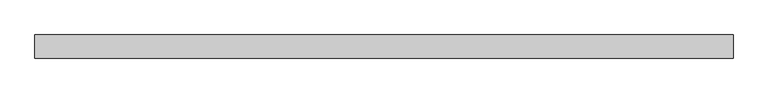
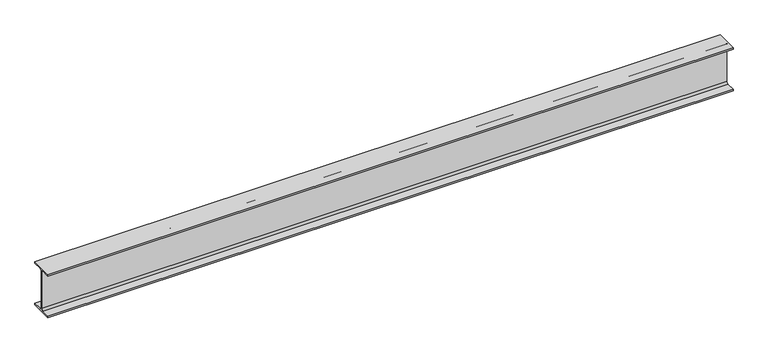
"""IFC4 building model written with IfcOpenShell, lengths in millimetres: beam geometry, 0912_Steel Framing_H-KSD3502 : H_SB_ASB_H-400x200x8x13."""

import ifcopenshell
import ifcopenshell.guid

model = None  # the IFC model being written
_history = None  # IfcOwnerHistory: only IFC2X3 demands one
_inside = {}  # id of a spatial element -> (the spatial element, [elements in it])
_under = {}  # id of a project, library or spatial element -> (it, [spatial elements below it])
_declared = {}  # id of a project -> (the project, [libraries it declares])
_typed = {}  # id of a type object -> (the type object, [elements of that type])
_made_of = {}  # id of a material, layer set ... -> (it, [elements and type objects made of it])


def new_model(schema):
    """Start an empty IFC model of exactly this schema.

    Asked for "IFC4X3", IfcOpenShell would pick the latest addendum, in which some entities
    have other attributes; the version numbers below select the first issue.
    IFC2X3 requires an IfcOwnerHistory on every rooted entity: one is made here for all.
    """
    global model, _history
    if schema == "IFC4X3":
        model = ifcopenshell.file(schema_version=(4, 3, 0, 0))
    else:
        model = ifcopenshell.file(schema=schema)
    _inside.clear()
    _under.clear()
    _declared.clear()
    _typed.clear()
    _made_of.clear()
    _history = None
    if model.schema == "IFC2X3":
        org = make("IfcOrganization", Name="unknown")
        user = make(
            "IfcPersonAndOrganization",
            ThePerson=make("IfcPerson", FamilyName="unknown"),
            TheOrganization=org,
        )
        app = make(
            "IfcApplication",
            ApplicationDeveloper=org,
            Version="unknown",
            ApplicationFullName="unknown",
            ApplicationIdentifier="unknown",
        )
        _history = make(
            "IfcOwnerHistory",
            OwningUser=user,
            OwningApplication=app,
            ChangeAction="ADDED",
            CreationDate=0,
        )
    return model


def make(cls, **values):
    """One entity of the class cls with the attributes given. An attribute that is None is left unset."""
    return model.create_entity(
        cls, **{name: value for name, value in values.items() if value is not None}
    )


def rooted(cls, **values):
    """An entity with a GlobalId (a new one), such as an element, a storey or a relation."""
    return make(cls, GlobalId=ifcopenshell.guid.new(), OwnerHistory=_history, **values)


def si_unit(unit_type, name, prefix=None):
    """IfcSIUnit, for example si_unit("LENGTHUNIT", "METRE", prefix="MILLI")."""
    return make("IfcSIUnit", UnitType=unit_type, Prefix=prefix, Name=name)


def assignment(units):
    """IfcUnitAssignment: the units of a project."""
    return None if units is None else make("IfcUnitAssignment", Units=units)


def point(xyz):
    """IfcCartesianPoint."""
    return None if xyz is None else make("IfcCartesianPoint", Coordinates=xyz)


def direction(xyz):
    """IfcDirection."""
    return None if xyz is None else make("IfcDirection", DirectionRatios=xyz)


def frame(location, z_axis=None, x_axis=None):
    """IfcAxis2Placement3D, a coordinate frame: its origin and axes. An axis left out is left unset."""
    return make(
        "IfcAxis2Placement3D",
        Location=point(location),
        Axis=direction(z_axis),
        RefDirection=direction(x_axis),
    )


def frame_2d(location, x_axis=None):
    """IfcAxis2Placement2D, a coordinate frame in the plane: its origin and x axis."""
    return make(
        "IfcAxis2Placement2D", Location=point(location), RefDirection=direction(x_axis)
    )


def origin():
    """The frame at (0, 0, 0) with its axes left unset."""
    return frame((0.0, 0.0, 0.0))


def place(relative_to, where):
    """IfcLocalPlacement: puts the frame where relative to a parent placement (None: the world)."""
    return make(
        "IfcLocalPlacement", PlacementRelTo=relative_to, RelativePlacement=where
    )


def context(
    kind, dimensions, precision=None, world=None, true_north=None, identifier=None
):
    """IfcGeometricRepresentationContext, for example the 3D "Model" context."""
    return make(
        "IfcGeometricRepresentationContext",
        ContextIdentifier=identifier,
        ContextType=kind,
        CoordinateSpaceDimension=dimensions,
        Precision=precision,
        WorldCoordinateSystem=world,
        TrueNorth=true_north,
    )


def project(units=None, contexts=None):
    """IfcProject with its units and contexts."""
    return rooted(
        "IfcProject",
        Name="project",
        RepresentationContexts=contexts,
        UnitsInContext=assignment(units),
    )


def spatial(cls, under=None, at=None, **own):
    """A site, building, storey or space (cls), placed at a placement, below another one or the project."""
    s = rooted(cls, ObjectPlacement=at, **own)
    if under is not None:
        _under.setdefault(under.id(), (under, []))[1].append(s)
    return s


def polyline(points):
    """IfcPolyline through the points."""
    return make("IfcPolyline", Points=[point(p) for p in points])


def circle_curve(where, radius):
    """IfcCircle in the frame where."""
    return make("IfcCircle", Position=where, Radius=radius)


def trimmed(basis, trim1, trim2, sense, master):
    """IfcTrimmedCurve: the piece of a basis curve between two trims."""
    return make(
        "IfcTrimmedCurve",
        BasisCurve=basis,
        Trim1=trim1,
        Trim2=trim2,
        SenseAgreement=sense,
        MasterRepresentation=master,
    )


def segment(curve, same_sense, transition):
    """IfcCompositeCurveSegment."""
    return make(
        "IfcCompositeCurveSegment",
        Transition=transition,
        SameSense=same_sense,
        ParentCurve=curve,
    )


def composite_curve(segments, self_intersect=None):
    """IfcCompositeCurve: segments joined end to end."""
    return make("IfcCompositeCurve", Segments=segments, SelfIntersect=self_intersect)


def outline(outer, holes=None, kind="AREA"):
    """IfcArbitraryClosedProfileDef: a profile drawn as a closed curve; with holes, ...WithVoids."""
    if holes is None:
        return make("IfcArbitraryClosedProfileDef", ProfileType=kind, OuterCurve=outer)
    return make(
        "IfcArbitraryProfileDefWithVoids",
        ProfileType=kind,
        OuterCurve=outer,
        InnerCurves=holes,
    )


def extrude(swept, where, along, depth):
    """IfcExtrudedAreaSolid: the profile swept, set in the frame where, extruded along a direction by depth."""
    return make(
        "IfcExtrudedAreaSolid",
        SweptArea=swept,
        Position=where,
        ExtrudedDirection=direction(along),
        Depth=depth,
    )


def shape(context_of_items, identifier, shape_type, items):
    """IfcShapeRepresentation: the items that make up one representation, for example the "Body"."""
    return make(
        "IfcShapeRepresentation",
        ContextOfItems=context_of_items,
        RepresentationIdentifier=identifier,
        RepresentationType=shape_type,
        Items=items,
    )


def source(mapping_origin, context_of_items, identifier, shape_type, items):
    """IfcRepresentationMap: a shape defined once, which mapped items show again and again."""
    return make(
        "IfcRepresentationMap",
        MappingOrigin=mapping_origin,
        MappedRepresentation=shape(context_of_items, identifier, shape_type, items),
    )


def transform(
    local_origin,
    x_axis=None,
    y_axis=None,
    z_axis=None,
    scale=None,
    scale2=None,
    scale3=None,
    uniform=True,
):
    """IfcCartesianTransformationOperator3D, or its non-uniform kind. x_axis, y_axis, z_axis: its Axis1, 2, 3."""
    if uniform:
        return make(
            "IfcCartesianTransformationOperator3D",
            Axis1=direction(x_axis),
            Axis2=direction(y_axis),
            LocalOrigin=point(local_origin),
            Scale=scale,
            Axis3=direction(z_axis),
        )
    return make(
        "IfcCartesianTransformationOperator3DnonUniform",
        Axis1=direction(x_axis),
        Axis2=direction(y_axis),
        LocalOrigin=point(local_origin),
        Scale=scale,
        Axis3=direction(z_axis),
        Scale2=scale2,
        Scale3=scale3,
    )


def mapped(mapping_source, mapping_target):
    """IfcMappedItem: shows the shape of a source again, moved by a transform."""
    return make(
        "IfcMappedItem", MappingSource=mapping_source, MappingTarget=mapping_target
    )


def made_of(thing, what):
    """Note that an element or type object is made of a material, layer set ...; save() writes the relation."""
    if what is not None:
        _made_of.setdefault(what.id(), (what, []))[1].append(thing)
    return thing


def element(
    cls,
    number,
    at=None,
    inside=None,
    cuts=None,
    type_object=None,
    material=None,
    context=None,
    identifier="Body",
    shape_type=None,
    held_by="IfcProductDefinitionShape",
    body=None,
    shapes=None,
    **own,
):
    """One element of the class cls, such as IfcWall. Its Tag is "e" and its number.

    at: its placement. inside: the storey or other place that contains it. cuts: it is an
    opening in that element (IfcRelVoidsElement). A single representation is given by context,
    identifier, shape_type and body (its items); several are given by shapes. held_by: the class
    of the entity that holds the representations. save() writes the other relations.
    """
    e = rooted(cls, Tag="e%d" % number, ObjectPlacement=at, **own)
    if body is not None:
        shapes = [shape(context, identifier, shape_type, body)]
    if shapes is not None:
        e.Representation = make(held_by, Representations=shapes)
    if inside is not None:
        _inside.setdefault(inside.id(), (inside, []))[1].append(e)
    if cuts is not None:
        rooted(
            "IfcRelVoidsElement", RelatingBuildingElement=cuts, RelatedOpeningElement=e
        )
    if type_object is not None:
        _typed.setdefault(type_object.id(), (type_object, []))[1].append(e)
    return made_of(e, material)


def aggregate(whole, parts):
    """IfcRelAggregates: a whole, such as a stair, and the parts it consists of."""
    return rooted("IfcRelAggregates", RelatingObject=whole, RelatedObjects=parts)


def save(model, path):
    """Write the relations noted so far, then the file.

    IfcRelAggregates (storeys below a building ...), IfcRelContainedInSpatialStructure (elements
    in a storey), IfcRelDefinesByType, IfcRelAssociatesMaterial and IfcRelDeclares: one each for
    every whole, place, type object, material and project.
    """
    for whole, parts in _under.values():
        aggregate(whole, parts)
    for where, things in _inside.values():
        rooted(
            "IfcRelContainedInSpatialStructure",
            RelatedElements=things,
            RelatingStructure=where,
        )
    for kind, things in _typed.values():
        rooted("IfcRelDefinesByType", RelatedObjects=things, RelatingType=kind)
    for what, things in _made_of.values():
        rooted("IfcRelAssociatesMaterial", RelatedObjects=things, RelatingMaterial=what)
    for by, libraries in _declared.values():
        rooted("IfcRelDeclares", RelatingContext=by, RelatedDefinitions=libraries)
    model.write(path)


def beam_f8e41749(model_context):
    return source(origin(), model_context, "Body", "SweptSolid", [
        extrude(outline(composite_curve([segment(polyline([(100.0, -187.0), (100.0, -200.0), (-100.0, -200.0), (-100.0, -187.0), (-20.0, -187.0)]), True, "CONTINUOUS"), segment(trimmed(circle_curve(frame_2d((-20.0, -171.0)), 16.0), [point((-20.0, -187.0))], [point((-4.0, -171.0))], True, "CARTESIAN"), True, "CONTINUOUS"), segment(polyline([(-4.0, -171.0), (-4.0, 171.0)]), True, "CONTINUOUS"), segment(trimmed(circle_curve(frame_2d((-20.0, 171.0)), 16.0), [point((-4.0, 171.0))], [point((-20.0, 187.0))], True, "CARTESIAN"), True, "CONTINUOUS"), segment(polyline([(-20.0, 187.0), (-100.0, 187.0), (-100.0, 200.0), (100.0, 200.0), (100.0, 187.0), (20.0, 187.0)]), True, "CONTINUOUS"), segment(trimmed(circle_curve(frame_2d((20.0, 171.0)), 16.0), [point((20.0, 187.0))], [point((4.0, 171.0))], True, "CARTESIAN"), True, "CONTINUOUS"), segment(polyline([(4.0, 171.0), (4.0, -171.0)]), True, "CONTINUOUS"), segment(trimmed(circle_curve(frame_2d((20.0, -171.0)), 16.0), [point((4.0, -171.0))], [point((20.0, -187.0))], True, "CARTESIAN"), True, "CONTINUOUS"), segment(polyline([(20.0, -187.0), (100.0, -187.0)]), True, "CONTINUOUS")], self_intersect=False)), frame((-3007.3488581, 0.0, 0.0), z_axis=(1.0, 0.0, 0.0), x_axis=(0.0, 1.0, 0.0)), (0.0, 0.0, 1.0), 6044.6488581),
    ])


if __name__ == "__main__":
    model = new_model("IFC4")
    model_context = context("Model", 3, world=origin())
    ifc_project = project(units=[si_unit("LENGTHUNIT", "METRE", prefix="MILLI")], contexts=[model_context])
    site = spatial("IfcSite", under=ifc_project)
    building = spatial("IfcBuilding", under=site)
    placement = place(None, origin())
    beam_shape = beam_f8e41749(model_context)
    element("IfcBeam", 1, ObjectType="0912_Steel Framing_H-KSD3502 : H_SB_ASB_H-400x200x8x13", at=placement, inside=building, context=model_context, shape_type="MappedRepresentation", body=[
        mapped(beam_shape, transform((0.0, 0.0, 0.0), x_axis=(1.0, 0.0, 0.0), y_axis=(0.0, 1.0, 0.0), z_axis=(0.0, 0.0, 1.0))),
    ])
    save(model, "model.ifc")

# Revit data of these elements
# Type "0912_Steel Framing_H-KSD3502 : H_SB_ASB_H-400x200x8x13"
#   H_WM Code_1 = "S01AA002-00001 | Main Steel Structure Fabrication Work | Shelter/Building | Medium Steel - Standard (90KG/M>Weight≥30KG/M) | Material: (   )"
#   H_WM Code_2 = "S03AA028-00001 | Main Steel Structure Erection Work | Shelter/Building | Medium Steel (90KG/M>Weight≥30KG/M) | Material: (   )"
#   H_WM Code_3 = "S01AA010-00001 | Main Steel Structure Fabrication Work | Shelter/Building | Steel Painting/Coating | for Non-Fireproofed Steel Surface, Surface Preparation, Primer, Second & Final Coat | Material: (   )"
#   H_Q'ty Cal Type Tag = "SB-Q2"
#   Width = 20.0 cm
#   Web Thickness = 0.8 cm
#   Web Fillet = 1.6 cm
#   Warping Constant = 649000.0 cm⁶
#   W = 0
#   Torsional Moment of Inertia = 35.8981 cm⁴
#   Section Area = 84.12 cm²
#   Plastic Modulus weak axis = 268.0 cm³
#   Plastic Modulus strong axis = 1330.0 cm³
#   Perimeter = 1.56 m²/m
#   Nominal Weight = 66.00 kgf/m
#   Moment of Inertia weak axis = 1740.00 cm⁴
#   Moment of Inertia strong axis = 23700.00 cm⁴
#   Height = 40.0 cm
#   Flange Thickness = 1.3 cm
#   Elastic Modulus weak axis = 174.0 cm³
#   Elastic Modulus strong axis = 1190.0 cm³
#   Centroid Vertical = 20.0 cm
#   Centroid Horizontal = 10.0 cm
#   Ix = 237000000
#   Length [instance default] = 1.5240 m
#   Zx = 1330000
#   b = 0.2000 m
#   h = 0.4000 m
#   r = 0.0160 m
#   s = 0.0080 m
#   t = 0.0130 m
#   A = 0.008412 m²
#   Structural Material [instance default] = Steel, 45-345
#   Assembly Code = ""
# Element 1 (IfcBeam, "0912_Steel Framing_H-KSD3502 : H_SB_ASB_H-400x200x8x13")
#   Structural Material = none
# Materials
#   "Steel, 45-345": class "Metal", colour RGB 189 187 185, transparency 0, Description = "Steel 345 MPa", Cost = 0
